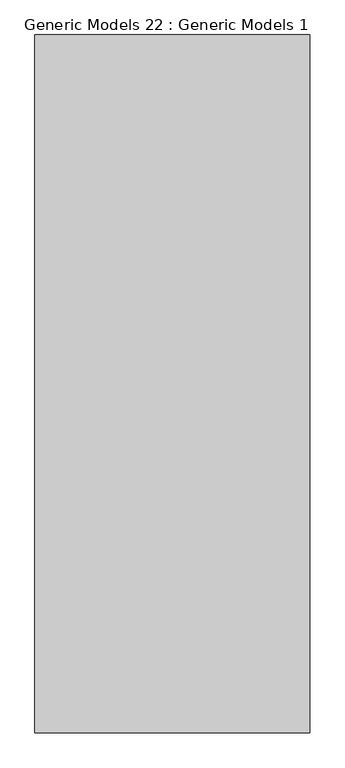
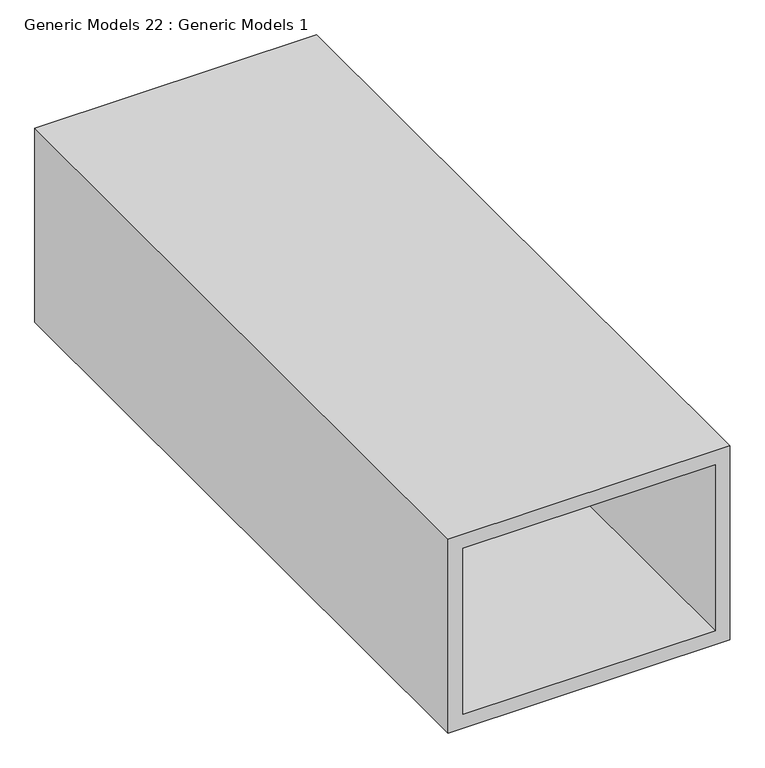
"""IFC4 building model written with IfcOpenShell, lengths in millimetres: proxy geometry, Generic Models 22 : Generic Models 1."""

import ifcopenshell
import ifcopenshell.guid

model = None  # the IFC model being written
_history = None  # IfcOwnerHistory: only IFC2X3 demands one
_inside = {}  # id of a spatial element -> (the spatial element, [elements in it])
_under = {}  # id of a project, library or spatial element -> (it, [spatial elements below it])
_declared = {}  # id of a project -> (the project, [libraries it declares])
_typed = {}  # id of a type object -> (the type object, [elements of that type])
_made_of = {}  # id of a material, layer set ... -> (it, [elements and type objects made of it])


def new_model(schema):
    """Start an empty IFC model of exactly this schema.

    Asked for "IFC4X3", IfcOpenShell would pick the latest addendum, in which some entities
    have other attributes; the version numbers below select the first issue.
    IFC2X3 requires an IfcOwnerHistory on every rooted entity: one is made here for all.
    """
    global model, _history
    if schema == "IFC4X3":
        model = ifcopenshell.file(schema_version=(4, 3, 0, 0))
    else:
        model = ifcopenshell.file(schema=schema)
    _inside.clear()
    _under.clear()
    _declared.clear()
    _typed.clear()
    _made_of.clear()
    _history = None
    if model.schema == "IFC2X3":
        org = make("IfcOrganization", Name="unknown")
        user = make(
            "IfcPersonAndOrganization",
            ThePerson=make("IfcPerson", FamilyName="unknown"),
            TheOrganization=org,
        )
        app = make(
            "IfcApplication",
            ApplicationDeveloper=org,
            Version="unknown",
            ApplicationFullName="unknown",
            ApplicationIdentifier="unknown",
        )
        _history = make(
            "IfcOwnerHistory",
            OwningUser=user,
            OwningApplication=app,
            ChangeAction="ADDED",
            CreationDate=0,
        )
    return model


def make(cls, **values):
    """One entity of the class cls with the attributes given. An attribute that is None is left unset."""
    return model.create_entity(
        cls, **{name: value for name, value in values.items() if value is not None}
    )


def rooted(cls, **values):
    """An entity with a GlobalId (a new one), such as an element, a storey or a relation."""
    return make(cls, GlobalId=ifcopenshell.guid.new(), OwnerHistory=_history, **values)


def si_unit(unit_type, name, prefix=None):
    """IfcSIUnit, for example si_unit("LENGTHUNIT", "METRE", prefix="MILLI")."""
    return make("IfcSIUnit", UnitType=unit_type, Prefix=prefix, Name=name)


def assignment(units):
    """IfcUnitAssignment: the units of a project."""
    return None if units is None else make("IfcUnitAssignment", Units=units)


def point(xyz):
    """IfcCartesianPoint."""
    return None if xyz is None else make("IfcCartesianPoint", Coordinates=xyz)


def direction(xyz):
    """IfcDirection."""
    return None if xyz is None else make("IfcDirection", DirectionRatios=xyz)


def frame(location, z_axis=None, x_axis=None):
    """IfcAxis2Placement3D, a coordinate frame: its origin and axes. An axis left out is left unset."""
    return make(
        "IfcAxis2Placement3D",
        Location=point(location),
        Axis=direction(z_axis),
        RefDirection=direction(x_axis),
    )


def origin():
    """The frame at (0, 0, 0) with its axes left unset."""
    return frame((0.0, 0.0, 0.0))


def place(relative_to, where):
    """IfcLocalPlacement: puts the frame where relative to a parent placement (None: the world)."""
    return make(
        "IfcLocalPlacement", PlacementRelTo=relative_to, RelativePlacement=where
    )


def context(
    kind, dimensions, precision=None, world=None, true_north=None, identifier=None
):
    """IfcGeometricRepresentationContext, for example the 3D "Model" context."""
    return make(
        "IfcGeometricRepresentationContext",
        ContextIdentifier=identifier,
        ContextType=kind,
        CoordinateSpaceDimension=dimensions,
        Precision=precision,
        WorldCoordinateSystem=world,
        TrueNorth=true_north,
    )


def project(units=None, contexts=None):
    """IfcProject with its units and contexts."""
    return rooted(
        "IfcProject",
        Name="project",
        RepresentationContexts=contexts,
        UnitsInContext=assignment(units),
    )


def spatial(cls, under=None, at=None, **own):
    """A site, building, storey or space (cls), placed at a placement, below another one or the project."""
    s = rooted(cls, ObjectPlacement=at, **own)
    if under is not None:
        _under.setdefault(under.id(), (under, []))[1].append(s)
    return s


def polyline(points):
    """IfcPolyline through the points."""
    return make("IfcPolyline", Points=[point(p) for p in points])


def outline(outer, holes=None, kind="AREA"):
    """IfcArbitraryClosedProfileDef: a profile drawn as a closed curve; with holes, ...WithVoids."""
    if holes is None:
        return make("IfcArbitraryClosedProfileDef", ProfileType=kind, OuterCurve=outer)
    return make(
        "IfcArbitraryProfileDefWithVoids",
        ProfileType=kind,
        OuterCurve=outer,
        InnerCurves=holes,
    )


def extrude(swept, where, along, depth):
    """IfcExtrudedAreaSolid: the profile swept, set in the frame where, extruded along a direction by depth."""
    return make(
        "IfcExtrudedAreaSolid",
        SweptArea=swept,
        Position=where,
        ExtrudedDirection=direction(along),
        Depth=depth,
    )


def shape(context_of_items, identifier, shape_type, items):
    """IfcShapeRepresentation: the items that make up one representation, for example the "Body"."""
    return make(
        "IfcShapeRepresentation",
        ContextOfItems=context_of_items,
        RepresentationIdentifier=identifier,
        RepresentationType=shape_type,
        Items=items,
    )


def source(mapping_origin, context_of_items, identifier, shape_type, items):
    """IfcRepresentationMap: a shape defined once, which mapped items show again and again."""
    return make(
        "IfcRepresentationMap",
        MappingOrigin=mapping_origin,
        MappedRepresentation=shape(context_of_items, identifier, shape_type, items),
    )


def transform(
    local_origin,
    x_axis=None,
    y_axis=None,
    z_axis=None,
    scale=None,
    scale2=None,
    scale3=None,
    uniform=True,
):
    """IfcCartesianTransformationOperator3D, or its non-uniform kind. x_axis, y_axis, z_axis: its Axis1, 2, 3."""
    if uniform:
        return make(
            "IfcCartesianTransformationOperator3D",
            Axis1=direction(x_axis),
            Axis2=direction(y_axis),
            LocalOrigin=point(local_origin),
            Scale=scale,
            Axis3=direction(z_axis),
        )
    return make(
        "IfcCartesianTransformationOperator3DnonUniform",
        Axis1=direction(x_axis),
        Axis2=direction(y_axis),
        LocalOrigin=point(local_origin),
        Scale=scale,
        Axis3=direction(z_axis),
        Scale2=scale2,
        Scale3=scale3,
    )


def mapped(mapping_source, mapping_target):
    """IfcMappedItem: shows the shape of a source again, moved by a transform."""
    return make(
        "IfcMappedItem", MappingSource=mapping_source, MappingTarget=mapping_target
    )


def made_of(thing, what):
    """Note that an element or type object is made of a material, layer set ...; save() writes the relation."""
    if what is not None:
        _made_of.setdefault(what.id(), (what, []))[1].append(thing)
    return thing


def element(
    cls,
    number,
    at=None,
    inside=None,
    cuts=None,
    type_object=None,
    material=None,
    context=None,
    identifier="Body",
    shape_type=None,
    held_by="IfcProductDefinitionShape",
    body=None,
    shapes=None,
    **own,
):
    """One element of the class cls, such as IfcWall. Its Tag is "e" and its number.

    at: its placement. inside: the storey or other place that contains it. cuts: it is an
    opening in that element (IfcRelVoidsElement). A single representation is given by context,
    identifier, shape_type and body (its items); several are given by shapes. held_by: the class
    of the entity that holds the representations. save() writes the other relations.
    """
    e = rooted(cls, Tag="e%d" % number, ObjectPlacement=at, **own)
    if body is not None:
        shapes = [shape(context, identifier, shape_type, body)]
    if shapes is not None:
        e.Representation = make(held_by, Representations=shapes)
    if inside is not None:
        _inside.setdefault(inside.id(), (inside, []))[1].append(e)
    if cuts is not None:
        rooted(
            "IfcRelVoidsElement", RelatingBuildingElement=cuts, RelatedOpeningElement=e
        )
    if type_object is not None:
        _typed.setdefault(type_object.id(), (type_object, []))[1].append(e)
    return made_of(e, material)


def aggregate(whole, parts):
    """IfcRelAggregates: a whole, such as a stair, and the parts it consists of."""
    return rooted("IfcRelAggregates", RelatingObject=whole, RelatedObjects=parts)


def save(model, path):
    """Write the relations noted so far, then the file.

    IfcRelAggregates (storeys below a building ...), IfcRelContainedInSpatialStructure (elements
    in a storey), IfcRelDefinesByType, IfcRelAssociatesMaterial and IfcRelDeclares: one each for
    every whole, place, type object, material and project.
    """
    for whole, parts in _under.values():
        aggregate(whole, parts)
    for where, things in _inside.values():
        rooted(
            "IfcRelContainedInSpatialStructure",
            RelatedElements=things,
            RelatingStructure=where,
        )
    for kind, things in _typed.values():
        rooted("IfcRelDefinesByType", RelatedObjects=things, RelatingType=kind)
    for what, things in _made_of.values():
        rooted("IfcRelAssociatesMaterial", RelatedObjects=things, RelatingMaterial=what)
    for by, libraries in _declared.values():
        rooted("IfcRelDeclares", RelatingContext=by, RelatedDefinitions=libraries)
    model.write(path)


def generic_models_22_generic_models_1_b0009ec1(model_context):
    return source(origin(), model_context, "Body", "SweptSolid", [
        extrude(outline(polyline([(2381.25, 51148.3797769), (2381.25, 50668.1069345), (2032.0, 50668.1069345), (2032.0, 51148.3797769), (2381.25, 51148.3797769)]), holes=[polyline([(2355.85, 51122.9797769), (2057.4, 51122.9797769), (2057.4, 50693.5069345), (2355.85, 50693.5069345), (2355.85, 51122.9797769)])]), frame((0.0, 0.0, 0.0), z_axis=(0.0, 1.0, 0.0), x_axis=(0.0, 0.0, 1.0)), (0.0, 0.0, 1.0), 1219.2),
    ])


if __name__ == "__main__":
    model = new_model("IFC4")
    model_context = context("Model", 3, world=origin())
    ifc_project = project(units=[si_unit("LENGTHUNIT", "METRE", prefix="MILLI")], contexts=[model_context])
    site = spatial("IfcSite", under=ifc_project)
    building = spatial("IfcBuilding", under=site)
    placement = place(None, origin())
    generic_models_22_generic_models_1_shape = generic_models_22_generic_models_1_b0009ec1(model_context)
    element("IfcBuildingElementProxy", 1, Name="Generic Models 22 : Generic Models 1", ObjectType="Generic Models 22 : Generic Models 1", at=placement, inside=building, context=model_context, shape_type="MappedRepresentation", body=[
        mapped(generic_models_22_generic_models_1_shape, transform((0.0, 0.0, 0.0), x_axis=(1.0, 0.0, 0.0), y_axis=(0.0, 1.0, 0.0), z_axis=(0.0, 0.0, 1.0))),
    ])
    save(model, "model.ifc")

# Revit data of these elements
# Element 1 (IfcBuildingElementProxy, "Generic Models 22 : Generic Models 1")
#   Materials on its faces: "IF THERE'S AN OPEN AIR WAY PATH, THROUGH THE DUCTS, FROM ONE ROOM TO THE OTHER, EITHER 1)LINE THE INTERIOR OF THE DUCT W/ SOUNDABSORPTIVE MATERIAL AND/OR 2) USE A 'DUCT BAFFLE BOX' TO MUFFLE THE MIGRATING SOUND"
# Materials
#   "IF THERE'S AN OPEN AIR WAY PATH, THROUGH THE DUCTS, FROM ONE ROOM TO THE OTHER, EITHER 1)LINE THE INTERIOR OF THE DUCT W/ SOUNDABSORPTIVE MATERIAL AND/OR 2) USE A 'DUCT BAFFLE BOX' TO MUFFLE THE MIGRATING SOUND": class "Generic", colour RGB 127 127 127, transparency 0, Description = "Rigid foam insulation board", Cost = 0
